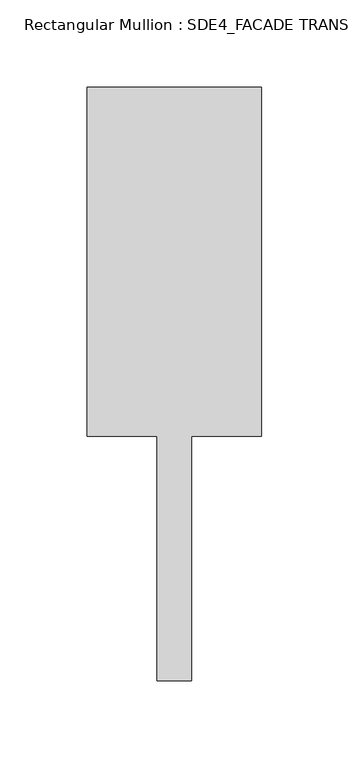
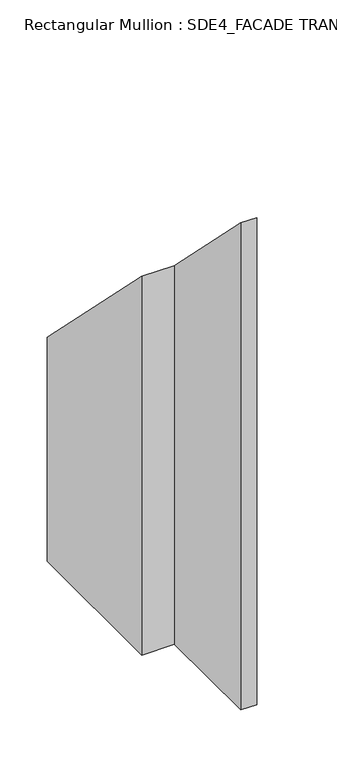
"""IFC4 building model written with IfcOpenShell, lengths in millimetres: member geometry, Rectangular Mullion : SDE4_FACADE TRANSOM TYPE 1."""

from ifc_helpers import new_model, si_unit, origin, place, context, project, spatial, faceted_brep, source, transform, mapped, element, save


def rectangular_mullion_sde4_facade_transom_type_1_a654ee0d(model_context):
    return source(origin(), model_context, "Body", "Brep", [
        faceted_brep([(50.0, 132.5, -421.9009563), (50.0, -67.5, -421.9009563), (10.0, -67.5, -421.9009563), (10.0, -207.5, -421.9009563), (-10.0, -207.5, -421.9009563), (-10.0, -67.5, -421.9009563), (-50.0, -67.5, -421.9009563), (-50.0, 132.5, -421.9009563), (-50.0, 132.5, -132.5), (50.0, 132.5, -132.5), (-50.0, -67.5, 67.5), (-10.0, -67.5, 67.5), (-10.0, -207.5, 207.5), (10.0, -207.5, 207.5), (10.0, -67.5, 67.5), (50.0, -67.5, 67.5)], [[[0, 1, 2, 3, 4, 5, 6, 7]], [[8, 9, 0, 7]], [[10, 8, 7, 6]], [[11, 10, 6, 5]], [[12, 11, 5, 4]], [[13, 12, 4, 3]], [[14, 13, 3, 2]], [[15, 14, 2, 1]], [[9, 15, 1, 0]], [[9, 8, 10, 11, 12, 13, 14, 15]]]),
    ])


if __name__ == "__main__":
    model = new_model("IFC4")
    model_context = context("Model", 3, world=origin())
    ifc_project = project(units=[si_unit("LENGTHUNIT", "METRE", prefix="MILLI")], contexts=[model_context])
    site = spatial("IfcSite", under=ifc_project)
    building = spatial("IfcBuilding", under=site)
    placement = place(None, origin())
    rectangular_mullion_sde4_facade_transom_type_1_shape = rectangular_mullion_sde4_facade_transom_type_1_a654ee0d(model_context)
    element("IfcMember", 1, ObjectType="Rectangular Mullion : SDE4_FACADE TRANSOM TYPE 1", at=placement, inside=building, context=model_context, shape_type="MappedRepresentation", body=[
        mapped(rectangular_mullion_sde4_facade_transom_type_1_shape, transform((0.0, 0.0, 0.0), x_axis=(1.0, 0.0, 0.0), y_axis=(0.0, 1.0, 0.0), z_axis=(0.0, 0.0, 1.0))),
    ])
    save(model, "model.ifc")

# Revit data of these elements
# Type "Rectangular Mullion : SDE4_FACADE TRANSOM TYPE 1"
#   built-in parameter 1007322 = 1.11549 (stored number, unit not read)
#   built-in parameter 1007321 = 0.164042 (stored number, unit not read)
#   built-in parameter 1007320 = 0.164042 (stored number, unit not read)
